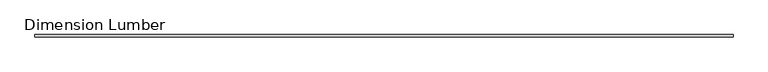
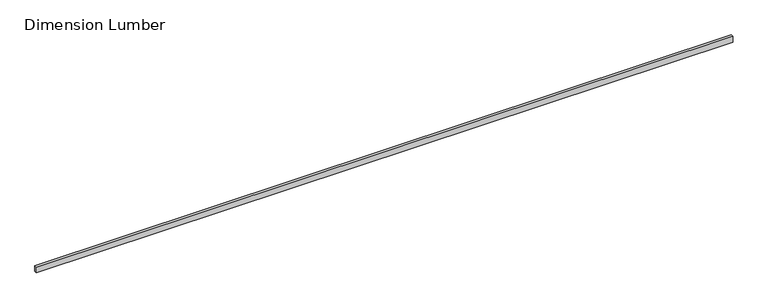
"""IFC4 building model written with IfcOpenShell, lengths in millimetres: beam geometry, Dimension Lumber : Roof Lumbers."""

from ifc_helpers import new_model, si_unit, frame, origin, place, context, project, spatial, polyline, outline, extrude, source, transform, mapped, element, save


def dimension_lumber_3c164bda(model_context):
    return source(origin(), model_context, "Body", "SweptSolid", [
        extrude(outline(polyline([(4638.675, -19.05), (-5762.625, -19.05), (-5762.625, 19.05), (4638.675, 19.05), (4638.675, -19.05)])), frame((0.0, 0.0, -44.45), z_axis=(0.0, 0.0, 1.0), x_axis=(1.0, 0.0, 0.0)), (0.0, 0.0, 1.0), 88.9),
    ])


if __name__ == "__main__":
    model = new_model("IFC4")
    model_context = context("Model", 3, world=origin())
    ifc_project = project(units=[si_unit("LENGTHUNIT", "METRE", prefix="MILLI")], contexts=[model_context])
    site = spatial("IfcSite", under=ifc_project)
    building = spatial("IfcBuilding", under=site)
    placement = place(None, origin())
    dimension_lumber_shape = dimension_lumber_3c164bda(model_context)
    element("IfcBeam", 1, ObjectType="Dimension Lumber : Roof Lumbers", at=placement, inside=building, context=model_context, shape_type="MappedRepresentation", body=[
        mapped(dimension_lumber_shape, transform((0.0, 0.0, 0.0), x_axis=(1.0, 0.0, 0.0), y_axis=(0.0, 1.0, 0.0), z_axis=(0.0, 0.0, 1.0))),
    ])
    save(model, "model.ifc")

# Revit data of these elements
# Type "Dimension Lumber : Roof Lumbers"
#   Assembly Code = "B10"
#   A = 0.0364583 SF
#   Length [instance default] = 5' - 0"
#   b = 0' - 1 1/2"
#   d = 0' - 3 1/2"
#   Structural Material [instance default] = Softwood, Lumber
# Element 1 (IfcBeam, "Dimension Lumber : Roof Lumbers")
#   Structural Material = Douglas Fir #2
#   Materials on its faces: "Douglas Fir #2"
# Materials
#   "Softwood, Lumber": class "Wood", colour RGB 223 192 134, transparency 0, Description = "Pinus Echinata", Cost = 0
#   "Douglas Fir #2": class "Wood", colour RGB 223 192 134, transparency 0, Description = "Pinus Echinata", Cost = 0
